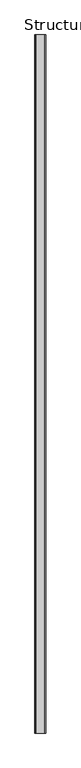
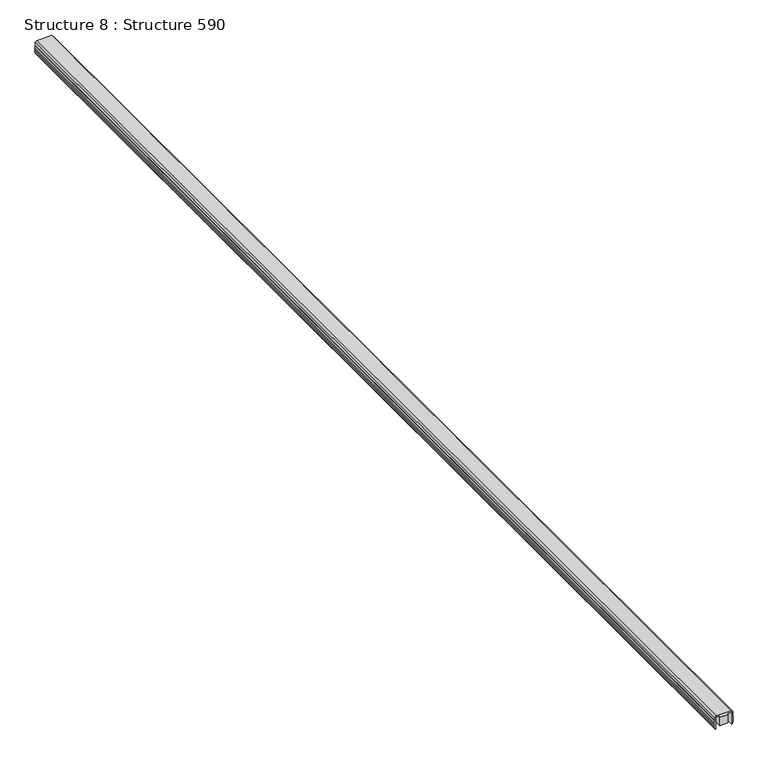
"""IFC4 building model written with IfcOpenShell, lengths in millimetres: proxy geometry, Structure 8 : Structure 590."""

from ifc_helpers import new_model, si_unit, frame, origin, place, context, project, spatial, polyline, outline, extrude, source, transform, mapped, element, save


def structure_8_structure_590_9bd57e5f(model_context):
    return source(origin(), model_context, "Body", "SweptSolid", [
        extrude(outline(polyline([(39518.6052323, 7622.5346434), (39516.0973628, 7620.0267738), (39511.2956147, 7620.0267738), (39509.4309187, 7620.5013448), (39506.7561917, 7619.6987269), (39506.7561917, 7620.5013448), (39504.0814647, 7619.6987269), (39504.0814647, 7620.5013448), (39501.4067377, 7619.6987269), (39501.4067377, 7620.5013448), (39498.7320107, 7619.6987269), (39498.7320107, 7620.5013448), (39496.0572836, 7620.5013448), (39494.2728422, 7622.2857862), (39515.9104029, 7622.2857862), (39515.9104029, 7628.6357862), (39513.3076045, 7628.6357862), (39513.3076045, 7642.4373027), (39515.9104029, 7642.4373027), (39515.9104029, 7648.7873027), (39494.2728422, 7648.7873027), (39496.0572836, 7650.5717441), (39498.7320107, 7650.5717441), (39498.7320107, 7651.374362), (39501.4067377, 7650.5717441), (39501.4067377, 7651.374362), (39504.0814647, 7650.5717441), (39504.0814647, 7651.374362), (39506.7561917, 7650.5717441), (39506.7561917, 7651.374362), (39509.4309187, 7650.5717441), (39511.2956147, 7651.0463151), (39516.0973628, 7651.0463151), (39518.6052323, 7648.5384455), (39518.6052323, 7622.5346434)])), frame((0.0, -3747.9491938, 0.0), z_axis=(0.0, 1.0, 0.0), x_axis=(0.0, 0.0, 1.0)), (0.0, 0.0, 1.0), 2000.0),
        extrude(outline(polyline([(7642.4373027, -3747.9491938), (7628.6357862, -3747.9491938), (7628.6357862, -1747.9491938), (7642.4373027, -1747.9491938), (7642.4373027, -3747.9491938)])), frame((0.0, 0.0, 39498.7320107), z_axis=(0.0, 0.0, 1.0), x_axis=(1.0, 0.0, 0.0)), (0.0, 0.0, 1.0), 14.5755939),
    ])


if __name__ == "__main__":
    model = new_model("IFC4")
    model_context = context("Model", 3, world=origin())
    ifc_project = project(units=[si_unit("LENGTHUNIT", "METRE", prefix="MILLI")], contexts=[model_context])
    site = spatial("IfcSite", under=ifc_project)
    building = spatial("IfcBuilding", under=site)
    placement = place(None, origin())
    structure_8_structure_590_shape = structure_8_structure_590_9bd57e5f(model_context)
    element("IfcBuildingElementProxy", 1, Name="Structure 8 : Structure 590", ObjectType="Structure 8 : Structure 590", at=placement, inside=building, context=model_context, shape_type="MappedRepresentation", body=[
        mapped(structure_8_structure_590_shape, transform((0.0, 0.0, 0.0), x_axis=(1.0, 0.0, 0.0), y_axis=(0.0, 1.0, 0.0), z_axis=(0.0, 0.0, 1.0))),
    ])
    save(model, "model.ifc")

# Revit data of these elements
# Type "Structure 8 : Structure 590"
#   NameOverride = "Structure"
# Element 1 (IfcBuildingElementProxy, "Structure 8 : Structure 590")
#   Materials on its faces: "RUBBER", "IfcSurfaceStyle #584"
# Materials
#   "RUBBER": class "Unassigned", colour RGB 70 70 70, transparency 0, Cost = 0
#   "IfcSurfaceStyle #584": class "Unassigned", colour RGB 169 181 186, transparency 0
